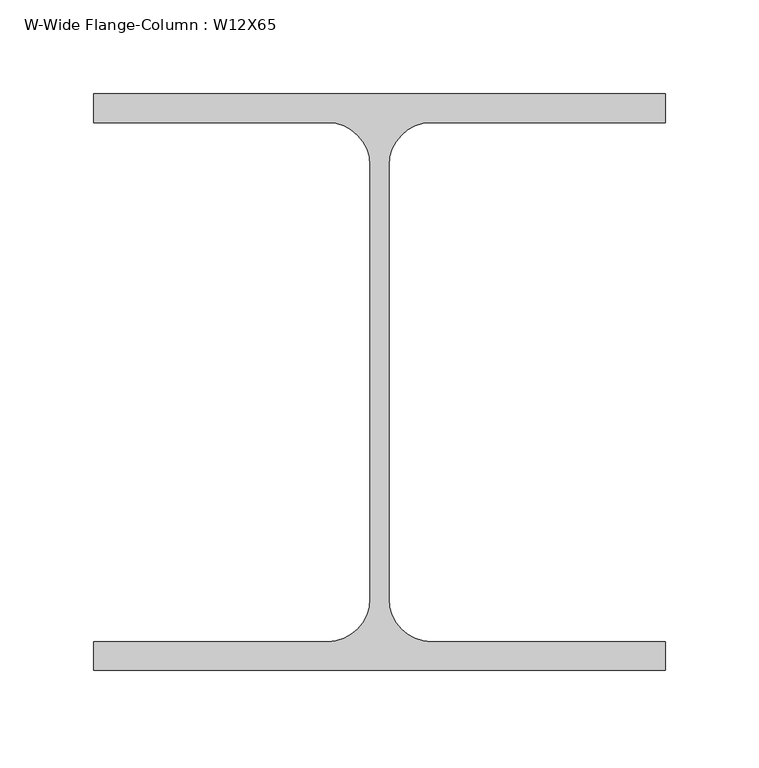
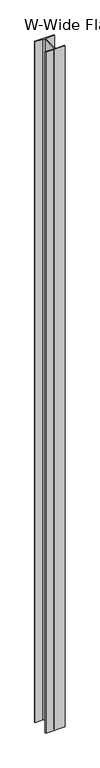
"""IFC4 building model written with IfcOpenShell, lengths in millimetres: column geometry, W-Wide Flange-Column : W12X65."""

from ifc_helpers import new_model, si_unit, point, frame, frame_2d, origin, place, context, project, spatial, polyline, circle_curve, trimmed, segment, composite_curve, outline, extrude, source, transform, mapped, element, save


def w_wide_flange_column_w12x65_65ba1ebc(model_context):
    return source(origin(), model_context, "Body", "SweptSolid", [
        extrude(outline(composite_curve([segment(polyline([(152.4, 153.67), (152.4, 138.303), (27.686, 138.303)]), True, "CONTINUOUS"), segment(trimmed(circle_curve(frame_2d((27.686, 115.57)), 22.733), [point((27.686, 138.303))], [point((4.953, 115.57))], True, "CARTESIAN"), True, "CONTINUOUS"), segment(polyline([(4.953, 115.57), (4.953, -115.57)]), True, "CONTINUOUS"), segment(trimmed(circle_curve(frame_2d((27.686, -115.57)), 22.733), [point((4.953, -115.57))], [point((27.686, -138.303))], True, "CARTESIAN"), True, "CONTINUOUS"), segment(polyline([(27.686, -138.303), (152.4, -138.303), (152.4, -153.67), (-152.4, -153.67), (-152.4, -138.303), (-27.686, -138.303)]), True, "CONTINUOUS"), segment(trimmed(circle_curve(frame_2d((-27.686, -115.57)), 22.733), [point((-27.686, -138.303))], [point((-4.953, -115.57))], True, "CARTESIAN"), True, "CONTINUOUS"), segment(polyline([(-4.953, -115.57), (-4.953, 115.57)]), True, "CONTINUOUS"), segment(trimmed(circle_curve(frame_2d((-27.686, 115.57)), 22.733), [point((-4.953, 115.57))], [point((-27.686, 138.303))], True, "CARTESIAN"), True, "CONTINUOUS"), segment(polyline([(-27.686, 138.303), (-152.4, 138.303), (-152.4, 153.67), (152.4, 153.67)]), True, "CONTINUOUS")], self_intersect=False)), frame((0.0, 0.0, 11849.1), z_axis=(0.0, 0.0, 1.0), x_axis=(1.0, 0.0, 0.0)), (0.0, 0.0, 1.0), 11468.1),
    ])


if __name__ == "__main__":
    model = new_model("IFC4")
    model_context = context("Model", 3, world=origin())
    ifc_project = project(units=[si_unit("LENGTHUNIT", "METRE", prefix="MILLI")], contexts=[model_context])
    site = spatial("IfcSite", under=ifc_project)
    building = spatial("IfcBuilding", under=site)
    placement = place(None, origin())
    w_wide_flange_column_w12x65_shape = w_wide_flange_column_w12x65_65ba1ebc(model_context)
    element("IfcColumn", 1, ObjectType="W-Wide Flange-Column : W12X65", at=placement, inside=building, context=model_context, shape_type="MappedRepresentation", body=[
        mapped(w_wide_flange_column_w12x65_shape, transform((0.0, 0.0, 0.0), x_axis=(1.0, 0.0, 0.0), y_axis=(0.0, 1.0, 0.0), z_axis=(0.0, 0.0, 1.0))),
    ])
    save(model, "model.ifc")

# Revit data of these elements
# Type "W-Wide Flange-Column : W12X65"
#   Assembly Code = "B10"
#   W = 65
#   bf = 1' - 0"
#   d = 1' - 0.1"
#   k = 0' - 1 1/2"
#   kr = 0' - 0.895"
#   tf = 0' - 0.605"
#   tw = 0' - 0.39"
#   A = 0.132639 SF
#   Structural Material [instance default] = Steel ASTM A992
# Element 1 (IfcColumn, "W-Wide Flange-Column : W12X65")
#   Materials on its faces: "Steel ASTM A992"
# Materials
#   "Steel ASTM A992": class "Metal", colour RGB 199 199 199, transparency 0, Description = "Structural steel 50ksi", Cost = 0
